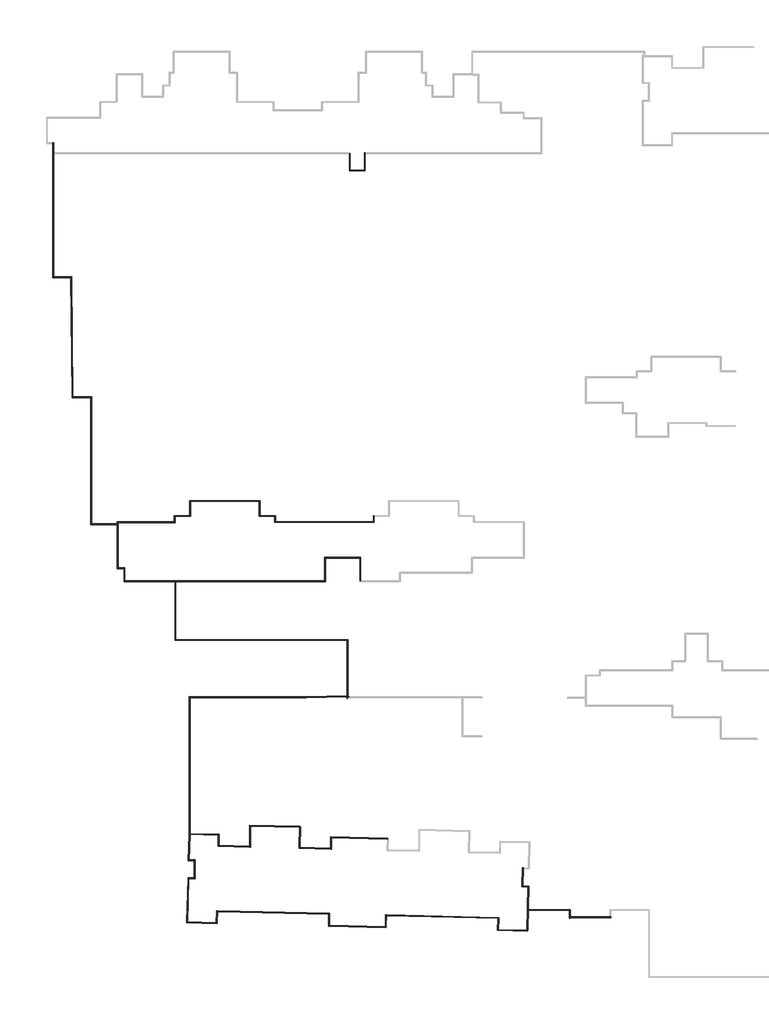
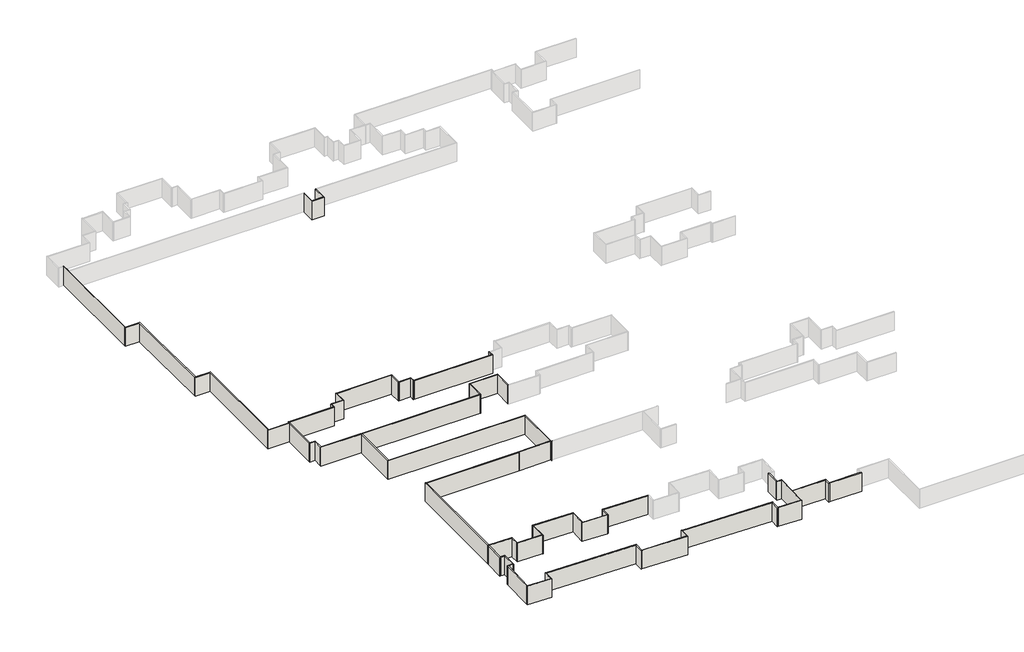
# One storey, part 1 of 8: 62 walls.
"""IFC4 building model written with IfcOpenShell, lengths in millimetres."""

from ifc_helpers import new_model, si_unit, origin, origin_with_axes, place, context, project, spatial, polyline, outline, extrude, faceted_brep, element, save

model = new_model("IFC4")

# Units and contexts
model_context = context("Model", 3, world=origin())
ifc_project = project(units=[si_unit("LENGTHUNIT", "METRE", prefix="MILLI")], contexts=[model_context])

# Site, building, storey
site = spatial("IfcSite", under=ifc_project)
building = spatial("IfcBuilding", under=site)
storey = spatial("IfcBuildingStorey", under=building, Name="户型图", Elevation=0.0)

# Walls
placement = place(None, origin())
element("IfcWall", 1, ObjectType="所有墙体", at=placement, inside=storey, context=model_context, shape_type="Brep", body=[
    faceted_brep([(102882.8943132, 25280.0239344, 0.0), (106917.4404066, 25139.1344803, 0.0), (106917.4404066, 25139.1344803, 3300.0), (102882.8943132, 25280.0239344, 3300.0), (102885.8292392, 25399.9945898, 0.0), (102885.8292392, 25399.9945898, 3300.0), (103005.7626841, 25395.8064217, 3300.0), (106801.7014469, 25263.2493191, 3300.0), (106921.6283462, 25259.0613795, 3300.0), (106921.6283462, 25259.0613795, 0.0), (106801.7014469, 25263.2493191, 0.0), (103005.7626841, 25395.8064217, 0.0)], [[[0, 1, 2, 3]], [[4, 5, 6, 7, 8, 9, 10, 11]], [[1, 0, 4, 11, 10, 9]], [[3, 2, 8, 7, 6, 5]], [[2, 1, 9, 8]], [[0, 3, 5, 4]]]),
])
element("IfcWall", 2, ObjectType="所有墙体", at=placement, inside=storey, context=model_context, shape_type="Brep", body=[
    faceted_brep([(106921.6283462, 25259.0613795, 0.0), (106974.697345, 26778.7586706, 0.0), (106978.8855131, 26898.6921155, 0.0), (106978.8855131, 26898.6921155, 3300.0), (106974.697345, 26778.7586706, 3300.0), (106921.6283462, 25259.0613795, 3300.0), (106801.7014469, 25263.2493191, 0.0), (106801.7014469, 25263.2493191, 3300.0), (106858.9148577, 26901.6270414, 3300.0), (106858.9148577, 26901.6270414, 0.0)], [[[0, 1, 2, 3, 4, 5]], [[6, 7, 8, 9]], [[2, 1, 0, 6, 9]], [[5, 4, 3, 8, 7]], [[0, 5, 7, 6]], [[3, 2, 9, 8]]]),
])
element("IfcWall", 3, ObjectType="所有墙体", at=placement, inside=storey, context=model_context, shape_type="Brep", body=[
    faceted_brep([(106974.697345, 26778.7586706, 0.0), (121834.0246766, 26415.2445642, 0.0), (121953.9887843, 26412.3097985, 0.0), (121953.9887843, 26412.3097985, 3300.0), (121834.0246766, 26415.2445642, 3300.0), (106974.697345, 26778.7586706, 3300.0), (106978.8855131, 26898.6921155, 0.0), (106978.8855131, 26898.6921155, 3300.0), (121956.9235501, 26532.2739062, 3300.0), (121956.9235501, 26532.2739062, 0.0)], [[[0, 1, 2, 3, 4, 5]], [[6, 7, 8, 9]], [[2, 1, 0, 6, 9]], [[5, 4, 3, 8, 7]], [[0, 5, 7, 6]], [[3, 2, 9, 8]]]),
])
element("IfcWall", 4, ObjectType="所有墙体", at=placement, inside=storey, context=model_context, shape_type="Brep", body=[
    faceted_brep([(121834.0246766, 26415.2445642, 0.0), (121794.8944661, 24815.7231259, 0.0), (121794.8944661, 24815.7231259, 3300.0), (121834.0246766, 26415.2445642, 3300.0), (121953.9887843, 26412.3097985, 0.0), (121953.9887843, 26412.3097985, 3300.0), (121917.7933396, 24932.7524679, 3300.0), (121914.8585738, 24812.7883601, 3300.0), (121914.8585738, 24812.7883601, 0.0), (121917.7933396, 24932.7524679, 0.0)], [[[0, 1, 2, 3]], [[4, 5, 6, 7, 8, 9]], [[1, 0, 4, 9, 8]], [[3, 2, 7, 6, 5]], [[0, 3, 5, 4]], [[2, 1, 8, 7]]]),
])
element("IfcWall", 5, ObjectType="所有墙体", at=placement, inside=storey, context=model_context, shape_type="Brep", body=[
    faceted_brep([(121914.8585738, 24812.7883601, 0.0), (129512.5853984, 24626.9198605, 0.0), (129512.5853984, 24626.9198605, 3300.0), (121914.8585738, 24812.7883601, 3300.0), (121917.7933396, 24932.7524679, 0.0), (121917.7933396, 24932.7524679, 3300.0), (129395.5560564, 24749.818734, 3300.0), (129515.5201642, 24746.8839682, 3300.0), (129515.5201642, 24746.8839682, 0.0), (129395.5560564, 24749.818734, 0.0)], [[[0, 1, 2, 3]], [[4, 5, 6, 7, 8, 9]], [[1, 0, 4, 9, 8]], [[3, 2, 7, 6, 5]], [[0, 3, 5, 4]], [[2, 1, 8, 7]]]),
])
element("IfcWall", 6, ObjectType="所有墙体", at=placement, inside=storey, context=model_context, shape_type="Brep", body=[
    faceted_brep([(129515.5201642, 24746.8839682, 0.0), (129551.7073968, 26226.1056131, 0.0), (129554.6421626, 26346.0697208, 0.0), (129554.6421626, 26346.0697208, 3300.0), (129551.7073968, 26226.1056131, 3300.0), (129515.5201642, 24746.8839682, 3300.0), (129395.5560564, 24749.818734, 0.0), (129395.5560564, 24749.818734, 3300.0), (129434.6780548, 26349.0044866, 3300.0), (129434.6780548, 26349.0044866, 0.0)], [[[0, 1, 2, 3, 4, 5]], [[6, 7, 8, 9]], [[2, 1, 0, 6, 9]], [[5, 4, 3, 8, 7]], [[0, 5, 7, 6]], [[3, 2, 9, 8]]]),
])
element("IfcWall", 7, ObjectType="所有墙体", at=placement, inside=storey, context=model_context, shape_type="Brep", body=[
    faceted_brep([(129551.7073968, 26226.1056131, 0.0), (144427.2567658, 25862.1946557, 0.0), (144547.2208736, 25859.2598899, 0.0), (144547.2208736, 25859.2598899, 3300.0), (144427.2567658, 25862.1946557, 3300.0), (129551.7073968, 26226.1056131, 3300.0), (129554.6421626, 26346.0697208, 0.0), (129554.6421626, 26346.0697208, 3300.0), (144550.1556394, 25979.2239977, 3300.0), (144550.1556394, 25979.2239977, 0.0)], [[[0, 1, 2, 3, 4, 5]], [[6, 7, 8, 9]], [[2, 1, 0, 6, 9]], [[5, 4, 3, 8, 7]], [[0, 5, 7, 6]], [[3, 2, 9, 8]]]),
])
element("IfcWall", 8, ObjectType="所有墙体", at=placement, inside=storey, context=model_context, shape_type="Brep", body=[
    faceted_brep([(144427.2567658, 25862.1946557, 0.0), (144388.1103472, 24262.0106797, 0.0), (144388.1103472, 24262.0106797, 3300.0), (144427.2567658, 25862.1946557, 3300.0), (144547.2208736, 25859.2598899, 0.0), (144547.2208736, 25859.2598899, 3300.0), (144511.0092207, 24379.0400217, 3300.0), (144508.074455, 24259.075914, 3300.0), (144508.074455, 24259.075914, 0.0), (144511.0092207, 24379.0400217, 0.0)], [[[0, 1, 2, 3]], [[4, 5, 6, 7, 8, 9]], [[1, 0, 4, 9, 8]], [[3, 2, 7, 6, 5]], [[0, 3, 5, 4]], [[2, 1, 8, 7]]]),
])
element("IfcWall", 9, ObjectType="所有墙体", at=placement, inside=storey, context=model_context, shape_type="Brep", body=[
    faceted_brep([(144508.074455, 24259.075914, 0.0), (148406.8372609, 24163.6977555, 0.0), (148406.8372609, 24163.6977555, 3300.0), (144508.074455, 24259.075914, 3300.0), (144511.0092207, 24379.0400217, 0.0), (144511.0092207, 24379.0400217, 3300.0), (148289.8079189, 24286.596629, 3300.0), (148409.7720267, 24283.6618632, 3300.0), (148409.7720267, 24283.6618632, 0.0), (148289.8079189, 24286.596629, 0.0)], [[[0, 1, 2, 3]], [[4, 5, 6, 7, 8, 9]], [[1, 0, 4, 9, 8]], [[3, 2, 7, 6, 5]], [[0, 3, 5, 4]], [[2, 1, 8, 7]]]),
])
element("IfcWall", 10, ObjectType="所有墙体", at=placement, inside=storey, context=model_context, shape_type="Brep", body=[
    faceted_brep([(148409.7720267, 24283.6618632, 0.0), (148554.0604637, 30181.7249031, 0.0), (148554.0604637, 30181.7249031, 3300.0), (148409.7720267, 24283.6618632, 3300.0), (148289.8079189, 24286.596629, 0.0), (148289.8079189, 24286.596629, 3300.0), (148431.1615901, 30064.6955611, 3300.0), (148434.0963559, 30184.6596688, 3300.0), (148434.0963559, 30184.6596688, 0.0), (148431.1615901, 30064.6955611, 0.0)], [[[0, 1, 2, 3]], [[4, 5, 6, 7, 8, 9]], [[1, 0, 4, 9, 8]], [[3, 2, 7, 6, 5]], [[0, 3, 5, 4]], [[2, 1, 8, 7]]]),
])
element("IfcWall", 11, ObjectType="所有墙体", at=placement, inside=storey, context=model_context, shape_type="Brep", body=[
    faceted_brep([(148434.0963559, 30184.6596688, 0.0), (147754.5603351, 30201.2836333, 0.0), (147634.5962273, 30204.2183991, 0.0), (147634.5962273, 30204.2183991, 3300.0), (147754.5603351, 30201.2836333, 3300.0), (148434.0963559, 30184.6596688, 3300.0), (148431.1615901, 30064.6955611, 0.0), (148431.1615901, 30064.6955611, 3300.0), (147631.6614615, 30084.2542913, 3300.0), (147631.6614615, 30084.2542913, 0.0)], [[[0, 1, 2, 3, 4, 5]], [[6, 7, 8, 9]], [[2, 1, 0, 6, 9]], [[5, 4, 3, 8, 7]], [[0, 5, 7, 6]], [[3, 2, 9, 8]]]),
])
element("IfcWall", 12, ObjectType="所有墙体", at=placement, inside=storey, context=model_context, shape_type="Brep", body=[
    faceted_brep([(147754.5603351, 30201.2836333, 0.0), (147810.3217494, 32480.6370168, 0.0), (147813.2565152, 32600.6011245, 0.0), (147813.2565152, 32600.6011245, 3300.0), (147810.3217494, 32480.6370168, 3300.0), (147754.5603351, 30201.2836333, 3300.0), (147634.5962273, 30204.2183991, 0.0), (147634.5962273, 30204.2183991, 3300.0), (147693.2924074, 32603.5358903, 3300.0), (147693.2924074, 32603.5358903, 0.0)], [[[0, 1, 2, 3, 4, 5]], [[6, 7, 8, 9]], [[2, 1, 0, 6, 9]], [[5, 4, 3, 8, 7]], [[0, 5, 7, 6]], [[3, 2, 9, 8]]]),
])
element("IfcWall", 13, ObjectType="所有墙体", at=placement, inside=storey, context=model_context, shape_type="Brep", body=[
    faceted_brep([(129684.1331467, 36545.953655, 0.0), (122084.9209931, 36731.8584912, 0.0), (122084.9209931, 36731.8584912, 3300.0), (129684.1331467, 36545.953655, 3300.0), (129681.1983809, 36425.9895472, 0.0), (129681.1983809, 36425.9895472, 3300.0), (122204.9209931, 36608.8869444, 3300.0), (122084.9209931, 36611.8225883, 3300.0), (122084.9209931, 36611.8225883, 0.0), (122204.9209931, 36608.8869444, 0.0)], [[[0, 1, 2, 3]], [[4, 5, 6, 7, 8, 9]], [[1, 0, 4, 9, 8]], [[3, 2, 7, 6, 5]], [[0, 3, 5, 4]], [[2, 1, 8, 7]]]),
])
element("IfcWall", 14, ObjectType="所有墙体", at=placement, inside=storey, context=model_context, shape_type="Brep", body=[
    faceted_brep([(122084.9209931, 36611.8225883, 0.0), (122084.9209931, 35231.8584912, 0.0), (122084.9209931, 35111.8225883, 0.0), (122084.9209931, 35111.8225883, 3300.0), (122084.9209931, 35231.8584912, 3300.0), (122084.9209931, 36611.8225883, 3300.0), (122204.9209931, 36608.8869444, 0.0), (122204.9209931, 36608.8869444, 3300.0), (122204.9209931, 35108.8869444, 3300.0), (122204.9209931, 35108.8869444, 0.0)], [[[0, 1, 2, 3, 4, 5]], [[6, 7, 8, 9]], [[2, 1, 0, 6, 9]], [[5, 4, 3, 8, 7]], [[0, 5, 7, 6]], [[3, 2, 9, 8]]]),
])
element("IfcWall", 15, ObjectType="所有墙体", at=placement, inside=storey, context=model_context, shape_type="Brep", body=[
    faceted_brep([(122084.9209931, 35231.8584912, 0.0), (118007.6266584, 35331.6041912, 0.0), (117887.6625506, 35334.538957, 0.0), (117887.6625506, 35334.538957, 3300.0), (118007.6266584, 35331.6041912, 3300.0), (122084.9209931, 35231.8584912, 3300.0), (122084.9209931, 35111.8225883, 0.0), (122084.9209931, 35111.8225883, 3300.0), (117884.7277848, 35214.5748493, 3300.0), (117884.7277848, 35214.5748493, 0.0)], [[[0, 1, 2, 3, 4, 5]], [[6, 7, 8, 9]], [[2, 1, 0, 6, 9]], [[5, 4, 3, 8, 7]], [[0, 5, 7, 6]], [[3, 2, 9, 8]]]),
])
element("IfcWall", 16, ObjectType="所有墙体", at=placement, inside=storey, context=model_context, shape_type="Brep", body=[
    faceted_brep([(118007.6266584, 35331.6041912, 0.0), (118076.08183, 38129.8389368, 0.0), (118076.08183, 38129.8389368, 3300.0), (118007.6266584, 35331.6041912, 3300.0), (117887.6625506, 35334.538957, 0.0), (117887.6625506, 35334.538957, 3300.0), (117953.1829565, 38012.8095948, 3300.0), (117956.1177223, 38132.7737026, 3300.0), (117956.1177223, 38132.7737026, 0.0), (117953.1829565, 38012.8095948, 0.0)], [[[0, 1, 2, 3]], [[4, 5, 6, 7, 8, 9]], [[1, 0, 4, 9, 8]], [[3, 2, 7, 6, 5]], [[0, 3, 5, 4]], [[2, 1, 8, 7]]]),
])
element("IfcWall", 17, ObjectType="所有墙体", at=placement, inside=storey, context=model_context, shape_type="Brep", body=[
    faceted_brep([(117956.1177223, 38132.7737026, 0.0), (111270.455721, 38296.3297232, 0.0), (111270.455721, 38296.3297232, 3300.0), (117956.1177223, 38132.7737026, 3300.0), (117953.1829565, 38012.8095948, 0.0), (117953.1829565, 38012.8095948, 3300.0), (111390.455721, 38173.3581764, 3300.0), (111270.455721, 38176.2938203, 3300.0), (111270.455721, 38176.2938203, 0.0), (111390.455721, 38173.3581764, 0.0)], [[[0, 1, 2, 3]], [[4, 5, 6, 7, 8, 9]], [[1, 0, 4, 9, 8]], [[3, 2, 7, 6, 5]], [[0, 3, 5, 4]], [[2, 1, 8, 7]]]),
])
element("IfcWall", 18, ObjectType="所有墙体", at=placement, inside=storey, context=model_context, shape_type="Brep", body=[
    faceted_brep([(111270.455721, 38176.2938203, 0.0), (111270.455721, 35496.3297232, 0.0), (111270.455721, 35376.2938203, 0.0), (111270.455721, 35376.2938203, 3300.0), (111270.455721, 35496.3297232, 3300.0), (111270.455721, 38176.2938203, 3300.0), (111390.455721, 38173.3581764, 0.0), (111390.455721, 38173.3581764, 3300.0), (111390.455721, 35373.3581764, 3300.0), (111390.455721, 35373.3581764, 0.0)], [[[0, 1, 2, 3, 4, 5]], [[6, 7, 8, 9]], [[2, 1, 0, 6, 9]], [[5, 4, 3, 8, 7]], [[0, 5, 7, 6]], [[3, 2, 9, 8]]]),
])
element("IfcWall", 19, ObjectType="所有墙体", at=placement, inside=storey, context=model_context, shape_type="Brep", body=[
    faceted_brep([(111270.455721, 35496.3297232, 0.0), (107191.7119495, 35596.1108818, 0.0), (107071.7119495, 35599.0465257, 0.0), (107071.7119495, 35599.0465257, 3300.0), (107191.7119495, 35596.1108818, 3300.0), (111270.455721, 35496.3297232, 3300.0), (111270.455721, 35376.2938203, 0.0), (111270.455721, 35376.2938203, 3300.0), (107071.7119495, 35479.0106227, 3300.0), (107071.7119495, 35479.0106227, 0.0)], [[[0, 1, 2, 3, 4, 5]], [[6, 7, 8, 9]], [[2, 1, 0, 6, 9]], [[5, 4, 3, 8, 7]], [[0, 5, 7, 6]], [[3, 2, 9, 8]]]),
])
element("IfcWall", 20, ObjectType="所有墙体", at=placement, inside=storey, context=model_context, shape_type="Brep", body=[
    faceted_brep([(107191.7119495, 35596.1108818, 0.0), (107191.7119495, 37096.1108818, 0.0), (107191.7119495, 37096.1108818, 3300.0), (107191.7119495, 35596.1108818, 3300.0), (107071.7119495, 35599.0465257, 0.0), (107071.7119495, 35599.0465257, 3300.0), (107071.7119495, 36979.0106227, 3300.0), (107071.7119495, 37099.0465257, 3300.0), (107071.7119495, 37099.0465257, 0.0), (107071.7119495, 36979.0106227, 0.0)], [[[0, 1, 2, 3]], [[4, 5, 6, 7, 8, 9]], [[1, 0, 4, 9, 8]], [[3, 2, 7, 6, 5]], [[0, 3, 5, 4]], [[2, 1, 8, 7]]]),
])
element("IfcWall", 21, ObjectType="所有墙体", at=placement, inside=storey, context=model_context, shape_type="Brep", body=[
    faceted_brep([(107071.7119495, 37099.0465257, 0.0), (103174.3637764, 37194.390077, 0.0), (103174.3637764, 37194.390077, 3300.0), (107071.7119495, 37099.0465257, 3300.0), (107071.7119495, 36979.0106227, 0.0), (107071.7119495, 36979.0106227, 3300.0), (103291.3931184, 37071.4912035, 3300.0), (103171.4290106, 37074.4259692, 3300.0), (103171.4290106, 37074.4259692, 0.0), (103291.3931184, 37071.4912035, 0.0)], [[[0, 1, 2, 3]], [[4, 5, 6, 7, 8, 9]], [[1, 0, 4, 9, 8]], [[3, 2, 7, 6, 5]], [[0, 3, 5, 4]], [[2, 1, 8, 7]]]),
])
element("IfcWall", 22, ObjectType="所有墙体", at=placement, inside=storey, context=model_context, shape_type="Brep", body=[
    faceted_brep([(103171.4290106, 37074.4259692, 0.0), (103085.7953386, 33573.9874973, 0.0), (103085.7953386, 33573.9874973, 3300.0), (103171.4290106, 37074.4259692, 3300.0), (103291.3931184, 37071.4912035, 0.0), (103291.3931184, 37071.4912035, 3300.0), (103208.7668855, 33693.9874973, 3300.0), (103205.8312416, 33573.9874973, 3300.0), (103205.8312416, 33573.9874973, 0.0), (103208.7668855, 33693.9874973, 0.0)], [[[0, 1, 2, 3]], [[4, 5, 6, 7, 8, 9]], [[1, 0, 4, 9, 8]], [[3, 2, 7, 6, 5]], [[0, 3, 5, 4]], [[2, 1, 8, 7]]]),
])
element("IfcWall", 23, ObjectType="所有墙体", at=placement, inside=storey, context=model_context, shape_type="Brep", body=[
    faceted_brep([(103205.8312416, 33573.9874973, 0.0), (103887.2811121, 33573.9874973, 0.0), (104007.2811121, 33573.9874973, 0.0), (104007.2811121, 33573.9874973, 3300.0), (103887.2811121, 33573.9874973, 3300.0), (103205.8312416, 33573.9874973, 3300.0), (103208.7668855, 33693.9874973, 0.0), (103208.7668855, 33693.9874973, 3300.0), (104007.2811121, 33693.9874973, 3300.0), (104007.2811121, 33693.9874973, 0.0)], [[[0, 1, 2, 3, 4, 5]], [[6, 7, 8, 9]], [[2, 1, 0, 6, 9]], [[5, 4, 3, 8, 7]], [[0, 5, 7, 6]], [[3, 2, 9, 8]]]),
])
element("IfcWall", 24, ObjectType="所有墙体", at=placement, inside=storey, context=model_context, shape_type="Brep", body=[
    faceted_brep([(103887.2811121, 33573.9874973, 0.0), (103887.2811121, 31274.9230596, 0.0), (103887.2811121, 31154.9230596, 0.0), (103887.2811121, 31154.9230596, 3300.0), (103887.2811121, 31274.9230596, 3300.0), (103887.2811121, 33573.9874973, 3300.0), (104007.2811121, 33573.9874973, 0.0), (104007.2811121, 33573.9874973, 3300.0), (104007.2811121, 31154.9230596, 3300.0), (104007.2811121, 31154.9230596, 0.0)], [[[0, 1, 2, 3, 4, 5]], [[6, 7, 8, 9]], [[2, 1, 0, 6, 9]], [[5, 4, 3, 8, 7]], [[0, 5, 7, 6]], [[3, 2, 9, 8]]]),
])
element("IfcWall", 25, ObjectType="所有墙体", at=placement, inside=storey, context=model_context, shape_type="Brep", body=[
    faceted_brep([(103887.2811121, 31274.9230596, 0.0), (103029.551719, 31274.9230596, 0.0), (103029.551719, 31274.9230596, 3300.0), (103887.2811121, 31274.9230596, 3300.0), (103887.2811121, 31154.9230596, 0.0), (103887.2811121, 31154.9230596, 3300.0), (103146.6519781, 31154.9230596, 3300.0), (103026.6160752, 31154.9230596, 3300.0), (103026.6160752, 31154.9230596, 0.0), (103146.6519781, 31154.9230596, 0.0)], [[[0, 1, 2, 3]], [[4, 5, 6, 7, 8, 9]], [[1, 0, 4, 9, 8]], [[3, 2, 7, 6, 5]], [[0, 3, 5, 4]], [[2, 1, 8, 7]]]),
])
element("IfcWall", 26, ObjectType="所有墙体", at=placement, inside=storey, context=model_context, shape_type="SweptSolid", body=[
    extrude(outline(polyline([(102885.8292392, 25399.9945898), (103026.6160752, 31154.9230596), (103146.6519781, 31154.9230596), (103005.7626841, 25395.8064217), (102885.8292392, 25399.9945898)])), origin_with_axes(), (0.0, 0.0, 1.0), 3300.0),
])
element("IfcWall", 27, ObjectType="所有墙体", at=placement, inside=storey, context=model_context, shape_type="Brep", body=[
    faceted_brep([(124375.3504625, 55452.5925367, 0.0), (124269.4925981, 55346.7346723, 0.0), (124269.4925981, 55346.7346723, 3300.0), (124375.3504625, 55452.5925367, 3300.0), (124545.05609, 55452.5925367, 0.0), (124545.05609, 55452.5925367, 3300.0), (124425.05609, 55332.5925367, 3300.0), (124269.4925981, 55177.0290448, 3300.0), (124269.4925981, 55177.0290448, 0.0), (124425.05609, 55332.5925367, 0.0)], [[[0, 1, 2, 3]], [[4, 5, 6, 7, 8, 9]], [[1, 0, 4, 9, 8]], [[3, 2, 7, 6, 5]], [[2, 1, 8, 7]], [[0, 3, 5, 4]]]),
])
element("IfcWall", 28, ObjectType="所有墙体", at=placement, inside=storey, context=model_context, shape_type="Brep", body=[
    faceted_brep([(124389.4925981, 55466.7346723, 0.0), (124389.4925981, 63081.8818585, 0.0), (124389.4925981, 63081.8818585, 3300.0), (124389.4925981, 55466.7346723, 3300.0), (124269.4925981, 55346.7346723, 0.0), (124269.4925981, 55346.7346723, 3300.0), (124269.4925981, 55479.0053901, 3300.0), (124269.4925981, 55599.0500099, 3300.0), (124269.4925981, 62961.8818585, 3300.0), (124269.4925981, 63081.8818585, 3300.0), (124269.4925981, 63081.8818585, 0.0), (124269.4925981, 62961.8818585, 0.0), (124269.4925981, 55599.0500099, 0.0), (124269.4925981, 55479.0053901, 0.0), (124375.3504625, 55452.5925367, 0.0), (124375.3504625, 55452.5925367, 3300.0)], [[[0, 1, 2, 3]], [[4, 5, 6, 7, 8, 9, 10, 11, 12, 13]], [[1, 0, 14, 4, 13, 12, 11, 10]], [[3, 2, 9, 8, 7, 6, 5, 15]], [[0, 3, 15, 5, 4, 14]], [[2, 1, 10, 9]]]),
])
element("IfcWall", 29, ObjectType="所有墙体", at=placement, inside=storey, context=model_context, shape_type="Brep", body=[
    faceted_brep([(124269.4925981, 63081.8818585, 0.0), (101409.5692161, 63081.8818585, 0.0), (101289.5692161, 63081.8818585, 0.0), (101289.5692161, 63081.8818585, 3300.0), (101409.5692161, 63081.8818585, 3300.0), (124269.4925981, 63081.8818585, 3300.0), (124269.4925981, 62961.8818585, 0.0), (124269.4925981, 62961.8818585, 3300.0), (101289.5692161, 62961.8818585, 3300.0), (101289.5692161, 62961.8818585, 0.0)], [[[0, 1, 2, 3, 4, 5]], [[6, 7, 8, 9]], [[2, 1, 0, 6, 9]], [[5, 4, 3, 8, 7]], [[0, 5, 7, 6]], [[3, 2, 9, 8]]]),
])
element("IfcWall", 30, ObjectType="所有墙体", at=placement, inside=storey, context=model_context, shape_type="SweptSolid", body=[
    extrude(outline(polyline([(101409.5692161, 70832.124524), (101409.5692161, 63081.8818585), (101289.5692161, 63081.8818585), (101289.5692161, 70832.1245314), (101409.5692161, 70832.124524)])), origin_with_axes(), (0.0, 0.0, 1.0), 3300.0),
])
element("IfcWall", 31, ObjectType="所有墙体", at=placement, inside=storey, context=model_context, shape_type="Brep", body=[
    faceted_brep([(121290.2513455, 70952.1233016, 0.0), (94610.165529, 70952.1249421, 0.0), (94490.165529, 70952.1249494, 0.0), (94490.165529, 70952.1249494, 3300.0), (94610.165529, 70952.1249421, 3300.0), (121290.2513455, 70952.1233016, 3300.0), (121290.2513455, 70832.1233016, 0.0), (121290.2513455, 70832.1233016, 3300.0), (101409.5692161, 70832.124524, 3300.0), (101289.5692161, 70832.1245314, 3300.0), (94490.165529, 70832.1249494, 3300.0), (94490.165529, 70832.1249494, 0.0), (101289.5692161, 70832.1245314, 0.0), (101409.5692161, 70832.124524, 0.0)], [[[0, 1, 2, 3, 4, 5]], [[6, 7, 8, 9, 10, 11, 12, 13]], [[2, 1, 0, 6, 13, 12, 11]], [[5, 4, 3, 10, 9, 8, 7]], [[3, 2, 11, 10]], [[0, 5, 7, 6]]]),
])
element("IfcWall", 32, ObjectType="所有墙体", at=placement, inside=storey, context=model_context, shape_type="Brep", body=[
    faceted_brep([(94610.165529, 70952.1249421, 0.0), (94610.165529, 72651.1555806, 0.0), (94610.165529, 72651.1555806, 3300.0), (94610.165529, 70952.1249421, 3300.0), (94490.165529, 70952.1249494, 0.0), (94490.165529, 70952.1249494, 3300.0), (94490.165529, 72531.1555806, 3300.0), (94490.165529, 72651.1555806, 3300.0), (94490.165529, 72651.1555806, 0.0), (94490.165529, 72531.1555806, 0.0)], [[[0, 1, 2, 3]], [[4, 5, 6, 7, 8, 9]], [[1, 0, 4, 9, 8]], [[3, 2, 7, 6, 5]], [[0, 3, 5, 4]], [[2, 1, 8, 7]]]),
])
element("IfcWall", 33, ObjectType="所有墙体", at=placement, inside=storey, context=model_context, shape_type="Brep", body=[
    faceted_brep([(94490.165529, 72651.1555806, 0.0), (93710.165529, 72651.1555806, 0.0), (93590.165529, 72651.1555806, 0.0), (93590.165529, 72651.1555806, 3300.0), (93710.165529, 72651.1555806, 3300.0), (94490.165529, 72651.1555806, 3300.0), (94490.165529, 72531.1555806, 0.0), (94490.165529, 72531.1555806, 3300.0), (93590.165529, 72531.1555806, 3300.0), (93590.165529, 72531.1555806, 0.0)], [[[0, 1, 2, 3, 4, 5]], [[6, 7, 8, 9]], [[2, 1, 0, 6, 9]], [[5, 4, 3, 8, 7]], [[0, 5, 7, 6]], [[3, 2, 9, 8]]]),
])
element("IfcWall", 34, ObjectType="所有墙体", at=placement, inside=storey, context=model_context, shape_type="Brep", body=[
    faceted_brep([(93710.165529, 72651.1555806, 0.0), (93710.165529, 78712.1296148, 0.0), (93710.165529, 78832.1296148, 0.0), (93710.165529, 78832.1296148, 3300.0), (93710.165529, 78712.1296148, 3300.0), (93710.165529, 72651.1555806, 3300.0), (93590.165529, 72651.1555806, 0.0), (93590.165529, 72651.1555806, 3300.0), (93590.165529, 78416.9697086, 3300.0), (93590.165529, 78536.9697086, 3300.0), (93590.165529, 78832.1296148, 3300.0), (93590.165529, 78832.1296148, 0.0), (93590.165529, 78536.9697086, 0.0), (93590.165529, 78416.9697086, 0.0)], [[[0, 1, 2, 3, 4, 5]], [[6, 7, 8, 9, 10, 11, 12, 13]], [[2, 1, 0, 6, 13, 12, 11]], [[5, 4, 3, 10, 9, 8, 7]], [[0, 5, 7, 6]], [[3, 2, 11, 10]]]),
])
element("IfcWall", 35, ObjectType="所有墙体", at=placement, inside=storey, context=model_context, shape_type="Brep", body=[
    faceted_brep([(93710.165529, 78712.1296148, 0.0), (101329.5692161, 78712.1296148, 0.0), (101329.5692161, 78712.1296148, 3300.0), (93710.165529, 78712.1296148, 3300.0), (93710.165529, 78832.1296148, 0.0), (93710.165529, 78832.1296148, 3300.0), (101209.5692161, 78832.1296148, 3300.0), (101329.5692161, 78832.1296148, 3300.0), (101329.5692161, 78832.1296148, 0.0), (101209.5692161, 78832.1296148, 0.0)], [[[0, 1, 2, 3]], [[4, 5, 6, 7, 8, 9]], [[1, 0, 4, 9, 8]], [[3, 2, 7, 6, 5]], [[0, 3, 5, 4]], [[2, 1, 8, 7]]]),
])
element("IfcWall", 36, ObjectType="所有墙体", at=placement, inside=storey, context=model_context, shape_type="Brep", body=[
    faceted_brep([(101329.5692161, 78832.1296148, 0.0), (101329.5692161, 79520.1923052, 0.0), (101329.5692161, 79640.1923052, 0.0), (101329.5692161, 79640.1923052, 3300.0), (101329.5692161, 79520.1923052, 3300.0), (101329.5692161, 78832.1296148, 3300.0), (101209.5692161, 78832.1296148, 0.0), (101209.5692161, 78832.1296148, 3300.0), (101209.5692161, 79640.1923052, 3300.0), (101209.5692161, 79640.1923052, 0.0)], [[[0, 1, 2, 3, 4, 5]], [[6, 7, 8, 9]], [[2, 1, 0, 6, 9]], [[5, 4, 3, 8, 7]], [[0, 5, 7, 6]], [[3, 2, 9, 8]]]),
])
element("IfcWall", 37, ObjectType="所有墙体", at=placement, inside=storey, context=model_context, shape_type="Brep", body=[
    faceted_brep([(101329.5692161, 79520.1923052, 0.0), (103359.1981527, 79520.1923052, 0.0), (103359.1981527, 79520.1923052, 3300.0), (101329.5692161, 79520.1923052, 3300.0), (101329.5692161, 79640.1923052, 0.0), (101329.5692161, 79640.1923052, 3300.0), (103239.1981527, 79640.1923052, 3300.0), (103359.1981527, 79640.1923052, 3300.0), (103359.1981527, 79640.1923052, 0.0), (103239.1981527, 79640.1923052, 0.0)], [[[0, 1, 2, 3]], [[4, 5, 6, 7, 8, 9]], [[1, 0, 4, 9, 8]], [[3, 2, 7, 6, 5]], [[0, 3, 5, 4]], [[2, 1, 8, 7]]]),
])
element("IfcWall", 38, ObjectType="所有墙体", at=placement, inside=storey, context=model_context, shape_type="Brep", body=[
    faceted_brep([(103359.1981527, 79640.1923052, 0.0), (103359.1981527, 81520.79875, 0.0), (103359.1981527, 81640.79875, 0.0), (103359.1981527, 81640.79875, 3300.0), (103359.1981527, 81520.79875, 3300.0), (103359.1981527, 79640.1923052, 3300.0), (103239.1981527, 79640.1923052, 0.0), (103239.1981527, 79640.1923052, 3300.0), (103239.1981527, 81640.79875, 3300.0), (103239.1981527, 81640.79875, 0.0)], [[[0, 1, 2, 3, 4, 5]], [[6, 7, 8, 9]], [[2, 1, 0, 6, 9]], [[5, 4, 3, 8, 7]], [[0, 5, 7, 6]], [[3, 2, 9, 8]]]),
])
element("IfcWall", 39, ObjectType="所有墙体", at=placement, inside=storey, context=model_context, shape_type="Brep", body=[
    faceted_brep([(103359.1981527, 81520.79875, 0.0), (112539.2356971, 81520.79875, 0.0), (112659.2356971, 81520.79875, 0.0), (112659.2356971, 81520.79875, 3300.0), (112539.2356971, 81520.79875, 3300.0), (103359.1981527, 81520.79875, 3300.0), (103359.1981527, 81640.79875, 0.0), (103359.1981527, 81640.79875, 3300.0), (112659.2356971, 81640.79875, 3300.0), (112659.2356971, 81640.79875, 0.0)], [[[0, 1, 2, 3, 4, 5]], [[6, 7, 8, 9]], [[2, 1, 0, 6, 9]], [[5, 4, 3, 8, 7]], [[0, 5, 7, 6]], [[3, 2, 9, 8]]]),
])
element("IfcWall", 40, ObjectType="所有墙体", at=placement, inside=storey, context=model_context, shape_type="Brep", body=[
    faceted_brep([(112539.2356971, 81520.79875, 0.0), (112539.2356971, 79520.1923052, 0.0), (112539.2356971, 79520.1923052, 3300.0), (112539.2356971, 81520.79875, 3300.0), (112659.2356971, 81520.79875, 0.0), (112659.2356971, 81520.79875, 3300.0), (112659.2356971, 79640.1923052, 3300.0), (112659.2356971, 79520.1923052, 3300.0), (112659.2356971, 79520.1923052, 0.0), (112659.2356971, 79640.1923052, 0.0)], [[[0, 1, 2, 3]], [[4, 5, 6, 7, 8, 9]], [[1, 0, 4, 9, 8]], [[3, 2, 7, 6, 5]], [[0, 3, 5, 4]], [[2, 1, 8, 7]]]),
])
element("IfcWall", 41, ObjectType="所有墙体", at=placement, inside=storey, context=model_context, shape_type="Brep", body=[
    faceted_brep([(112659.2356971, 79520.1923052, 0.0), (114589.266717, 79520.1923052, 0.0), (114709.266717, 79520.1923052, 0.0), (114709.266717, 79520.1923052, 3300.0), (114589.266717, 79520.1923052, 3300.0), (112659.2356971, 79520.1923052, 3300.0), (112659.2356971, 79640.1923052, 0.0), (112659.2356971, 79640.1923052, 3300.0), (114709.266717, 79640.1923052, 3300.0), (114709.266717, 79640.1923052, 0.0)], [[[0, 1, 2, 3, 4, 5]], [[6, 7, 8, 9]], [[2, 1, 0, 6, 9]], [[5, 4, 3, 8, 7]], [[0, 5, 7, 6]], [[3, 2, 9, 8]]]),
])
element("IfcWall", 42, ObjectType="所有墙体", at=placement, inside=storey, context=model_context, shape_type="Brep", body=[
    faceted_brep([(114589.266717, 79520.1923052, 0.0), (114589.266717, 78721.1444171, 0.0), (114589.266717, 78721.1444171, 3300.0), (114589.266717, 79520.1923052, 3300.0), (114709.266717, 79520.1923052, 0.0), (114709.266717, 79520.1923052, 3300.0), (114709.266717, 78841.1444171, 3300.0), (114709.266717, 78721.1444171, 3300.0), (114709.266717, 78721.1444171, 0.0), (114709.266717, 78841.1444171, 0.0)], [[[0, 1, 2, 3]], [[4, 5, 6, 7, 8, 9]], [[1, 0, 4, 9, 8]], [[3, 2, 7, 6, 5]], [[0, 3, 5, 4]], [[2, 1, 8, 7]]]),
])
element("IfcWall", 43, ObjectType="所有墙体", at=placement, inside=storey, context=model_context, shape_type="Brep", body=[
    faceted_brep([(114709.266717, 78721.1444171, 0.0), (127910.0897862, 78721.1444171, 0.0), (127910.0897862, 78721.1444171, 3300.0), (114709.266717, 78721.1444171, 3300.0), (114709.266717, 78841.1444171, 0.0), (114709.266717, 78841.1444171, 3300.0), (127790.0897862, 78841.1444171, 3300.0), (127910.0897862, 78841.1444171, 3300.0), (127910.0897862, 78841.1444171, 0.0), (127790.0897862, 78841.1444171, 0.0)], [[[0, 1, 2, 3]], [[4, 5, 6, 7, 8, 9]], [[1, 0, 4, 9, 8]], [[3, 2, 7, 6, 5]], [[0, 3, 5, 4]], [[2, 1, 8, 7]]]),
])
element("IfcWall", 44, ObjectType="所有墙体", at=placement, inside=storey, context=model_context, shape_type="Brep", body=[
    faceted_brep([(127910.0897862, 78841.1444171, 0.0), (127910.0897862, 79520.2608397, 0.0), (127910.0897862, 79640.2608397, 0.0), (127910.0897862, 79640.2608397, 3300.0), (127910.0897862, 79520.2608397, 3300.0), (127910.0897862, 78841.1444171, 3300.0), (127790.0897862, 78841.1444171, 0.0), (127790.0897862, 78841.1444171, 3300.0), (127790.0897862, 79640.2608397, 3300.0), (127790.0897862, 79640.2608397, 0.0)], [[[0, 1, 2, 3, 4, 5]], [[6, 7, 8, 9]], [[2, 1, 0, 6, 9]], [[5, 4, 3, 8, 7]], [[0, 5, 7, 6]], [[3, 2, 9, 8]]]),
])
element("IfcWall", 45, ObjectType="所有墙体", at=placement, inside=storey, context=model_context, shape_type="Brep", body=[
    faceted_brep([(126110.2513394, 70952.1232979, 0.0), (126110.2513394, 74052.1202767, 0.0), (126110.2513394, 74052.1202767, 3300.0), (126110.2513394, 70952.1232979, 3300.0), (125990.2513394, 70952.1232979, 0.0), (125990.2513394, 70952.1232979, 3300.0), (125990.2513394, 73932.1202767, 3300.0), (125990.2513394, 74052.1202767, 3300.0), (125990.2513394, 74052.1202767, 0.0), (125990.2513394, 73932.1202767, 0.0)], [[[0, 1, 2, 3]], [[4, 5, 6, 7, 8, 9]], [[1, 0, 4, 9, 8]], [[3, 2, 7, 6, 5]], [[0, 3, 5, 4]], [[2, 1, 8, 7]]]),
])
element("IfcWall", 46, ObjectType="所有墙体", at=placement, inside=storey, context=model_context, shape_type="Brep", body=[
    faceted_brep([(125990.2513394, 74052.1202767, 0.0), (121290.2513455, 74052.1202767, 0.0), (121290.2513455, 74052.1202767, 3300.0), (125990.2513394, 74052.1202767, 3300.0), (125990.2513394, 73932.1202767, 0.0), (125990.2513394, 73932.1202767, 3300.0), (121410.2513455, 73932.1202767, 3300.0), (121290.2513455, 73932.1202767, 3300.0), (121290.2513455, 73932.1202767, 0.0), (121410.2513455, 73932.1202767, 0.0)], [[[0, 1, 2, 3]], [[4, 5, 6, 7, 8, 9]], [[1, 0, 4, 9, 8]], [[3, 2, 7, 6, 5]], [[0, 3, 5, 4]], [[2, 1, 8, 7]]]),
])
element("IfcWall", 47, ObjectType="所有墙体", at=placement, inside=storey, context=model_context, shape_type="Brep", body=[
    faceted_brep([(121290.2513455, 73932.1202767, 0.0), (121290.2513455, 70952.1233016, 0.0), (121290.2513455, 70832.1233016, 0.0), (121290.2513455, 70832.1233016, 3300.0), (121290.2513455, 70952.1233016, 3300.0), (121290.2513455, 73932.1202767, 3300.0), (121410.2513455, 73932.1202767, 0.0), (121410.2513455, 73932.1202767, 3300.0), (121410.2513455, 70832.1232942, 3300.0), (121410.2513455, 70832.1232942, 0.0), (121398.8557829, 70832.1232949, 3300.0)], [[[0, 1, 2, 3, 4, 5]], [[6, 7, 8, 9]], [[2, 1, 0, 6, 9]], [[5, 4, 3, 10, 8, 7]], [[0, 5, 7, 6]], [[3, 2, 9, 8, 10]]]),
])
element("IfcWall", 48, ObjectType="所有墙体", at=placement, inside=storey, context=model_context, shape_type="Brep", body=[
    faceted_brep([(93590.165529, 78536.9697086, 0.0), (90160.3013005, 78536.9697086, 0.0), (90040.3013005, 78536.9697086, 0.0), (90040.3013005, 78536.9697086, 3300.0), (90160.3013005, 78536.9697086, 3300.0), (93590.165529, 78536.9697086, 3300.0), (93590.165529, 78416.9697086, 0.0), (93590.165529, 78416.9697086, 3300.0), (90040.3013005, 78416.9697086, 3300.0), (90040.3013005, 78416.9697086, 0.0)], [[[0, 1, 2, 3, 4, 5]], [[6, 7, 8, 9]], [[2, 1, 0, 6, 9]], [[5, 4, 3, 8, 7]], [[0, 5, 7, 6]], [[3, 2, 9, 8]]]),
])
element("IfcWall", 49, ObjectType="所有墙体", at=placement, inside=storey, context=model_context, shape_type="Brep", body=[
    faceted_brep([(90160.3013005, 78536.9697086, 0.0), (90160.3013005, 95477.3846604, 0.0), (90160.3013005, 95477.3846604, 3300.0), (90160.3013005, 78536.9697086, 3300.0), (90040.3013005, 78536.9697086, 0.0), (90040.3013005, 78536.9697086, 3300.0), (90040.3013005, 95357.3846604, 3300.0), (90040.3013005, 95477.3846604, 3300.0), (90040.3013005, 95477.3846604, 0.0), (90040.3013005, 95357.3846604, 0.0)], [[[0, 1, 2, 3]], [[4, 5, 6, 7, 8, 9]], [[1, 0, 4, 9, 8]], [[3, 2, 7, 6, 5]], [[0, 3, 5, 4]], [[2, 1, 8, 7]]]),
])
element("IfcWall", 50, ObjectType="所有墙体", at=placement, inside=storey, context=model_context, shape_type="Brep", body=[
    faceted_brep([(90040.3013005, 95477.3846604, 0.0), (87659.7435193, 95477.3846604, 0.0), (87539.7382853, 95477.3846604, 0.0), (87539.7382853, 95477.3846604, 3300.0), (87659.7435193, 95477.3846604, 3300.0), (90040.3013005, 95477.3846604, 3300.0), (90040.3013005, 95357.3846604, 0.0), (90040.3013005, 95357.3846604, 3300.0), (87540.8590816, 95357.3846604, 3300.0), (87540.8590816, 95357.3846604, 0.0)], [[[0, 1, 2, 3, 4, 5]], [[6, 7, 8, 9]], [[2, 1, 0, 6, 9]], [[5, 4, 3, 8, 7]], [[0, 5, 7, 6]], [[3, 2, 9, 8]]]),
])
element("IfcWall", 51, ObjectType="所有墙体", at=placement, inside=storey, context=model_context, shape_type="Brep", body=[
    faceted_brep([(87659.7435193, 95477.3846604, 0.0), (87509.7435642, 111537.3894148, 0.0), (87509.7435642, 111537.3894148, 2700.0), (87509.7435642, 111537.3894148, 3300.0), (87555.9297135, 106592.3894162, 3300.0), (87650.3009381, 96488.3709529, 3300.0), (87659.7435193, 95477.3846604, 3300.0), (87659.7435193, 95477.3846604, 2700.0), (87539.7382853, 95477.3846604, 0.0), (87539.7382853, 95477.3846604, 3300.0), (87390.8591266, 111417.3894148, 3300.0), (87389.7383302, 111537.3894148, 3300.0), (87389.7383302, 111537.3894148, 0.0), (87390.8591266, 111417.3894148, 0.0), (87450.3009381, 111537.3894148, 3300.0)], [[[0, 1, 2, 3, 4, 5, 6, 7]], [[8, 9, 10, 11, 12, 13]], [[1, 0, 8, 13, 12]], [[6, 5, 4, 3, 14, 11, 10, 9]], [[0, 7, 6, 9, 8]], [[3, 2, 1, 12, 11, 14]]]),
])
element("IfcWall", 52, ObjectType="所有墙体", at=placement, inside=storey, context=model_context, shape_type="Brep", body=[
    faceted_brep([(87389.7383302, 111537.3894148, 0.0), (85110.3013454, 111537.3894148, 0.0), (84990.3013454, 111537.3894148, 0.0), (84990.3013454, 111537.3894148, 3300.0), (85110.3013454, 111537.3894148, 3300.0), (87389.7383302, 111537.3894148, 3300.0), (87390.8591266, 111417.3894148, 0.0), (87390.8591266, 111417.3894148, 3300.0), (84990.3013454, 111417.3894148, 3300.0), (84990.3013454, 111417.3894148, 0.0)], [[[0, 1, 2, 3, 4, 5]], [[6, 7, 8, 9]], [[2, 1, 0, 6, 9]], [[5, 4, 3, 8, 7]], [[0, 5, 7, 6]], [[3, 2, 9, 8]]]),
])
element("IfcWall", 53, ObjectType="所有墙体", at=placement, inside=storey, context=model_context, shape_type="Brep", body=[
    faceted_brep([(85110.3013454, 111537.3894148, 0.0), (85110.3013454, 127947.6292793, 0.0), (85110.3013454, 128067.6292793, 0.0), (85110.3013454, 129402.6292795, 0.0), (85110.3013454, 129402.6292795, 3300.0), (85110.3013454, 128067.6292793, 3300.0), (85110.3013454, 127947.6292793, 3300.0), (85110.3013454, 111537.3894148, 3300.0), (84990.3013454, 111537.3894148, 0.0), (84990.3013454, 111537.3894148, 3300.0), (84990.3013454, 129282.6292795, 3300.0), (84990.3013454, 129402.6292795, 3300.0), (84990.3013454, 129402.6292795, 0.0), (84990.3013454, 129282.6292795, 0.0)], [[[0, 1, 2, 3, 4, 5, 6, 7]], [[8, 9, 10, 11, 12, 13]], [[3, 2, 1, 0, 8, 13, 12]], [[7, 6, 5, 4, 11, 10, 9]], [[0, 7, 9, 8]], [[4, 3, 12, 11]]]),
])
element("IfcWall", 54, ObjectType="所有墙体", at=placement, inside=storey, context=model_context, shape_type="Brep", body=[
    faceted_brep([(124590.5968759, 127947.6292793, 0.0), (124590.5968759, 125647.6292794, 0.0), (124590.5968759, 125647.6292794, 2700.0), (124590.5968759, 125647.6292794, 3300.0), (124590.5968759, 125767.6292794, 3300.0), (124590.5968759, 127947.6292793, 3300.0), (124710.5968759, 127947.6292793, 0.0), (124710.5968759, 127947.6292793, 3300.0), (124710.5968759, 125767.6292794, 3300.0), (124710.5968759, 125647.6292794, 3300.0), (124710.5968759, 125647.6292794, 0.0), (124710.5968759, 125767.6292794, 0.0)], [[[0, 1, 2, 3, 4, 5]], [[6, 7, 8, 9, 10, 11]], [[1, 0, 6, 11, 10]], [[5, 4, 3, 9, 8, 7]], [[0, 5, 7, 6]], [[3, 2, 1, 10, 9]]]),
])
element("IfcWall", 55, ObjectType="所有墙体", at=placement, inside=storey, context=model_context, shape_type="Brep", body=[
    faceted_brep([(124710.5968759, 125647.6292794, 0.0), (126709.8101643, 125647.6292794, 0.0), (126709.8101643, 125647.6292794, 3300.0), (124710.5968759, 125647.6292794, 3300.0), (124710.5968759, 125767.6292794, 0.0), (124710.5968759, 125767.6292794, 3300.0), (126589.8101643, 125767.6292794, 3300.0), (126709.8101643, 125767.6292794, 3300.0), (126709.8101643, 125767.6292794, 0.0), (126589.8101643, 125767.6292794, 0.0)], [[[0, 1, 2, 3]], [[4, 5, 6, 7, 8, 9]], [[1, 0, 4, 9, 8]], [[3, 2, 7, 6, 5]], [[0, 3, 5, 4]], [[2, 1, 8, 7]]]),
])
element("IfcWall", 56, ObjectType="所有墙体", at=placement, inside=storey, context=model_context, shape_type="Brep", body=[
    faceted_brep([(126709.8101643, 125767.6292794, 0.0), (126709.8101643, 127947.6292793, 0.0), (126709.8101643, 128067.6292793, 0.0), (126709.8101643, 128067.6292793, 3300.0), (126709.8101643, 127947.6292793, 3300.0), (126709.8101643, 125767.6292794, 3300.0), (126589.8101643, 125767.6292794, 0.0), (126589.8101643, 125767.6292794, 3300.0), (126589.8101643, 128067.6292793, 3300.0), (126589.8101643, 128067.6292793, 0.0)], [[[0, 1, 2, 3, 4, 5]], [[6, 7, 8, 9]], [[2, 1, 0, 6, 9]], [[5, 4, 3, 8, 7]], [[0, 5, 7, 6]], [[3, 2, 9, 8]]]),
])
element("IfcWall", 57, ObjectType="所有墙体", at=placement, inside=storey, context=model_context, shape_type="Brep", body=[
    faceted_brep([(148474.3885407, 26924.9842098, 0.0), (153972.7804968, 26924.9842098, 0.0), (154092.7804968, 26924.9842098, 0.0), (154092.7804968, 26924.9842098, 3300.0), (153972.7804968, 26924.9842098, 3300.0), (148474.3885407, 26924.9842098, 3300.0), (148477.3241845, 27044.9842098, 0.0), (148477.3241845, 27044.9842098, 3300.0), (154092.7804968, 27044.9842098, 3300.0), (154092.7804968, 27044.9842098, 0.0)], [[[0, 1, 2, 3, 4, 5]], [[6, 7, 8, 9]], [[2, 1, 0, 6, 9]], [[5, 4, 3, 8, 7]], [[3, 2, 9, 8]], [[0, 5, 7, 6]]]),
])
element("IfcWall", 58, ObjectType="所有墙体", at=placement, inside=storey, context=model_context, shape_type="Brep", body=[
    faceted_brep([(153972.7804968, 26924.9842098, 0.0), (153972.7804968, 25884.9842098, 0.0), (153972.7804968, 25884.9842098, 3300.0), (153972.7804968, 26924.9842098, 3300.0), (154092.7804968, 26924.9842098, 0.0), (154092.7804968, 26924.9842098, 3300.0), (154092.7804968, 26052.2214543, 3300.0), (154092.7804968, 25932.2214543, 3300.0), (154092.7804968, 25884.9842098, 3300.0), (154092.7804968, 25884.9842098, 0.0), (154092.7804968, 25932.2214543, 0.0), (154092.7804968, 26052.2214543, 0.0)], [[[0, 1, 2, 3]], [[4, 5, 6, 7, 8, 9, 10, 11]], [[1, 0, 4, 11, 10, 9]], [[2, 1, 9, 8]], [[3, 2, 8, 7, 6, 5]], [[0, 3, 5, 4]]]),
])
element("IfcWall", 59, ObjectType="所有墙体", at=placement, inside=storey, context=model_context, shape_type="Brep", body=[
    faceted_brep([(154092.7804968, 25932.2214543, 0.0), (159492.7804968, 25932.2214543, 0.0), (159492.7804968, 25932.2214543, 3300.0), (154092.7804968, 25932.2214543, 3300.0), (154092.7804968, 26052.2214543, 0.0), (154092.7804968, 26052.2214543, 3300.0), (159372.7804968, 26052.2214543, 3300.0), (159492.7804968, 26052.2214543, 3300.0), (159492.7804968, 26052.2214543, 0.0), (159372.7804968, 26052.2214543, 0.0)], [[[0, 1, 2, 3]], [[4, 5, 6, 7, 8, 9]], [[1, 0, 4, 9, 8]], [[3, 2, 7, 6, 5]], [[0, 3, 5, 4]], [[2, 1, 8, 7]]]),
])
element("IfcWall", 60, ObjectType="所有墙体", at=placement, inside=storey, context=model_context, shape_type="Brep", body=[
    faceted_brep([(103292.8784474, 37191.4907698, 0.0), (103292.8784474, 55332.5925366, 0.0), (103292.8784474, 55452.5925366, 0.0), (103292.8784474, 55452.5925366, 3300.0), (103292.8784474, 55332.5925366, 3300.0), (103292.8784474, 55092.5925366, 3300.0), (103292.8784474, 38806.8951488, 3300.0), (103292.8784474, 37191.4907698, 3300.0), (103292.8784474, 37191.4907698, 2700.0), (103172.8784474, 37194.4264136, 0.0), (103172.8784474, 37194.4264136, 2700.0), (103172.8784474, 37194.4264136, 3300.0), (103172.8784474, 38806.8951488, 3300.0), (103172.8784474, 55092.5925366, 3300.0), (103172.8784474, 55392.5925366, 3300.0), (103172.8784474, 55452.5925366, 3300.0), (103172.8784474, 55452.5925366, 0.0)], [[[0, 1, 2, 3, 4, 5, 6, 7, 8]], [[9, 10, 11, 12, 13, 14, 15, 16]], [[2, 1, 0, 9, 16]], [[7, 6, 5, 4, 3, 15, 14, 13, 12, 11]], [[3, 2, 16, 15]], [[0, 8, 7, 11, 10, 9]]]),
])
element("IfcWall", 61, ObjectType="所有墙体", at=placement, inside=storey, context=model_context, shape_type="Brep", body=[
    faceted_brep([(103292.8784474, 55332.5925366, 0.0), (118901.021306, 55332.5925366, 0.0), (118901.021306, 55332.5925366, 3300.0), (118750.2032763, 55332.5925366, 3300.0), (103292.8784474, 55332.5925366, 3300.0), (103292.8784474, 55332.5925366, 2700.0), (103292.8784474, 55452.5925366, 0.0), (103292.8784474, 55452.5925366, 3300.0), (118899.3852465, 55452.5925366, 3300.0), (118899.3852465, 55452.5925366, 0.0)], [[[0, 1, 2, 3, 4, 5]], [[6, 7, 8, 9]], [[1, 0, 6, 9]], [[4, 3, 2, 8, 7]], [[0, 5, 4, 7, 6]], [[2, 1, 9, 8]]]),
])
element("IfcWall", 62, ObjectType="所有墙体", at=placement, inside=storey, context=model_context, shape_type="Brep", body=[
    faceted_brep([(118901.021306, 55332.5925366, 0.0), (124269.4925981, 55479.0053901, 0.0), (124269.4925981, 55479.0053901, 3300.0), (123522.2775593, 55458.6267981, 3300.0), (119050.2032763, 55336.6611358, 3300.0), (118901.021306, 55332.5925366, 3300.0), (118899.3852465, 55452.5925366, 0.0), (118899.3852465, 55452.5925366, 3300.0), (124269.4925981, 55599.0500099, 3300.0), (124269.4925981, 55599.0500099, 0.0)], [[[0, 1, 2, 3, 4, 5]], [[6, 7, 8, 9]], [[1, 0, 6, 9]], [[5, 4, 3, 2, 8, 7]], [[0, 5, 7, 6]], [[2, 1, 9, 8]]]),
])

save(model, "model.ifc")

# Revit data of these elements
# Project information
#   项目发布日期 = "出图日期"
#   项目状态 = "项目状态"
#   客户姓名 = "所有者"
#   项目地址 = "## 街道\n省市自治区邮政编码"
#   项目名称 = "项目名称"
#   项目编号 = "项目编号"
# Type "所有墙体"
#   Layers, outside or top first: 120 mm "默认" (function 1)
# Elements 1, 2, 3, 4, 5, 6, 7, 8, 9, 10, 11, 12, 13, 14, 15, 16, 17, 18, 19, 20, 21, 22, 23, 24, 25, 26, 27, 28, 29, 30, 31, 32, 33, 34, 35, 36, 37, 38, 39, 40, 41, 42, 43, 44, 45, 46, 47 (IfcWall, "所有墙体")
#   Top Offset = 0 mm
#   Base Offset = 0 mm
#   wall height = 3300 mm
#   Phase Created = 新构造
#   Base Constraint = 户型图
#   Top Constraint = 层高
#   Materials on its faces: "默认"
# Elements 48, 49, 50, 51, 52, 53, 54, 55, 56, 57, 58, 59, 60, 61, 62 (IfcWall, "所有墙体")
#   Comments = ""
#   Top Offset = 0 mm
#   Base Offset = 0 mm
#   wall height = 3300 mm
#   Phase Created = 新构造
#   Base Constraint = 户型图
#   Top Constraint = 层高
#   Materials on its faces: "默认"
# Materials
#   "默认": class "其他", colour RGB 192 192 192, transparency 0, Cost = 0
# Area at (118429.314, 131484.863) mm, upper offset 0 mm, lower offset 0 mm
#   Number = "9"
#   Name = "main_building"
# Area at (190072.526, 134514.794) mm, upper offset 0 mm, lower offset 0 mm
#   Number = "10"
#   Name = "main_building"
# Area at (273346.764, 131484.863) mm, upper offset 0 mm, lower offset 0 mm
#   Number = "11"
#   Name = "main_building"
# Area at (170820.268, 96195.326) mm, upper offset 0 mm, lower offset 0 mm
#   Number = "12"
#   Name = "main_building"
# Area at (204635.414, 95189.912) mm, upper offset 0 mm, lower offset 0 mm
#   Number = "13"
#   Name = "main_building"
# Area at (240743.168, 98264.619) mm, upper offset 0 mm, lower offset 0 mm
#   Number = "14"
#   Name = "main_building"
# Area at (276344.959, 98264.619) mm, upper offset 0 mm, lower offset 0 mm
#   Number = "15"
#   Name = "main_building"
# Area at (302436.731, 98948.727) mm, upper offset 0 mm, lower offset 0 mm
#   Number = "16"
#   Name = "main_building"
# Area at (297583.405, 57735.776) mm, upper offset 0 mm, lower offset 0 mm
#   Number = "17"
#   Name = "main_building"
# Area at (240307.768, 56175.217) mm, upper offset 0 mm, lower offset 0 mm
#   Number = "18"
#   Name = "main_building"
# Area at (240307.768, 56175.217) mm, upper offset 0 mm, lower offset 0 mm
#   Number = "19"
#   Name = "面积"
# Area at (171969.324, 56175.217) mm, upper offset 0 mm, lower offset 0 mm
#   Number = "20"
#   Name = "main_building"
# Area at (276344.959, 19911.35) mm, upper offset 0 mm, lower offset 0 mm
#   Number = "21"
#   Name = "main_building"
# Area at (127122.221, 30589.414) mm, upper offset 0 mm, lower offset 0 mm
#   Number = "22"
#   Name = "main_building"
# Room, not placed, phase "新构造", upper offset 0 mm, lower offset 0 mm
#   Number = "9"
#   Name = "客餐厅轮廓"
# Room, not placed, phase "新构造", upper offset 0 mm, lower offset 0 mm
#   Number = "10"
#   Name = "墙面轮廓"
# Area at (258225.684, 39396.103) mm, upper offset 0 mm, lower offset 0 mm
#   Number = "6"
#   Name = "fire_compart_4"
# Room, not placed, phase "新构造", upper offset 0 mm, lower offset 0 mm
#   Number = "1"
#   Name = "客餐厅"
# Room, not placed, phase "新构造", upper offset 0 mm, lower offset 0 mm
#   Number = "2"
#   Name = "阳台"
# Room, not placed, phase "新构造", upper offset 0 mm, lower offset 0 mm
#   Number = "3"
#   Name = "次卧"
# Room, not placed, phase "新构造", upper offset 0 mm, lower offset 0 mm
#   Number = "4"
#   Name = "厨房"
# Room, not placed, phase "新构造", upper offset 0 mm, lower offset 0 mm
#   Number = "5"
#   Name = "卫生间"
# Room, not placed, phase "新构造", upper offset 0 mm, lower offset 0 mm
#   Number = "6"
#   Name = "次卧"
# Room, not placed, phase "新构造", upper offset 0 mm, lower offset 0 mm
#   Number = "7"
#   Name = "主卧"
# Area at (116597.856, 75701.69) mm, upper offset 0 mm, lower offset 0 mm
#   Number = "23"
#   Name = "main_building"
# Area at (234520.364, 77531.792) mm, upper offset 0 mm, lower offset 0 mm
#   Number = "7"
#   Name = "fire_compart_5"
# Area, not placed, upper offset 0 mm, lower offset 0 mm
#   Number = "1"
#   Name = "面积"
# Area, not placed, upper offset 0 mm, lower offset 0 mm
#   Number = "2"
#   Name = "防火区域1"
# Room, not placed, phase "新构造", upper offset 0 mm, lower offset 0 mm
#   Number = "8"
#   Name = "客餐厅"
# Area at (243896.331, 112697.282) mm, upper offset 0 mm, lower offset 0 mm
#   Number = "8"
#   Name = "fire_compart_6"
# Area at (133288.233, 110855.854) mm, upper offset 0 mm, lower offset 0 mm
#   Number = "3"
#   Name = "fire_compart_1"
# Room, not placed, phase "新构造", upper offset 0 mm, lower offset 0 mm
#   Number = "11"
#   Name = "房间"
# Room, not placed, phase "新构造", upper offset 0 mm, lower offset 0 mm
#   Number = "12"
#   Name = "房间"
# Room, not placed, phase "新构造", upper offset 0 mm, lower offset 0 mm
#   Number = "13"
#   Name = "房间"
# Room, not placed, phase "新构造", upper offset 0 mm, lower offset 0 mm
#   Number = "14"
#   Name = "房间"
# Room, not placed, phase "新构造", upper offset 0 mm, lower offset 0 mm
#   Number = "15"
#   Name = "房间"
# Room, not placed, phase "新构造", upper offset 0 mm, lower offset 0 mm
#   Number = "16"
#   Name = "房间"
# Room, not placed, phase "新构造", upper offset 0 mm, lower offset 0 mm
#   Number = "17"
#   Name = "房间"
# Area at (157450.33, 39681.103) mm, upper offset 0 mm, lower offset 0 mm
#   Number = "5"
#   Name = "fire_compart_3"
# Area at (155632.78, 75199.167) mm, upper offset 0 mm, lower offset 0 mm
#   Number = "4"
#   Name = "fire_compart_2"
